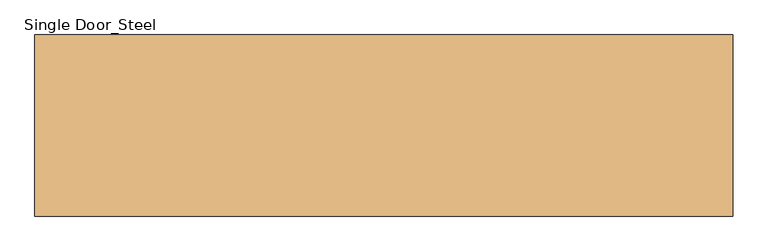
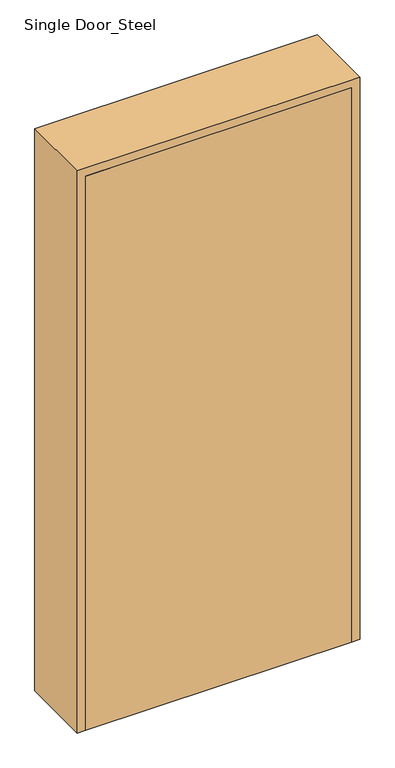
"""IFC4 building model written with IfcOpenShell, lengths in millimetres: door geometry, Single Door_Steel : H_DR_AR_B12_Single Door_Steel_W1000xH2100."""

from ifc_helpers import new_model, si_unit, origin, origin_with_axes, place, context, project, spatial, polyline, outline, extrude, faceted_brep, source, transform, mapped, element, save


def single_door_steel_02f153ad(model_context):
    return source(origin(), model_context, "Body", "SolidModel", [
        extrude(outline(polyline([(470.0, -130.0), (-470.0, -130.0), (-470.0, -95.0), (470.0, -95.0), (470.0, -130.0)])), origin_with_axes(), (0.0, 0.0, 1.0), 2070.0),
        faceted_brep([(470.0, -130.0, 0.0), (470.0, -95.0, 0.0), (450.0, -95.0, 0.0), (450.0, 95.0, 0.0), (470.0, 95.0, 0.0), (470.0, 130.0, 0.0), (500.0, 130.0, 0.0), (500.0, -130.0, 0.0), (500.0, -130.0, 2100.0), (-500.0, -130.0, 2100.0), (-500.0, -130.0, 0.0), (-470.0, -130.0, 0.0), (-470.0, -130.0, 2070.0), (470.0, -130.0, 2070.0), (500.0, 130.0, 2100.0), (470.0, 130.0, 2070.0), (-470.0, 130.0, 2070.0), (-470.0, 130.0, 0.0), (-500.0, 130.0, 0.0), (-500.0, 130.0, 2100.0), (470.0, 95.0, 2070.0), (450.0, 95.0, 2050.0), (-450.0, 95.0, 2050.0), (-450.0, 95.0, 0.0), (-470.0, 95.0, 0.0), (-470.0, 95.0, 2070.0), (450.0, -95.0, 2050.0), (470.0, -95.0, 2070.0), (-470.0, -95.0, 2070.0), (-470.0, -95.0, 0.0), (-450.0, -95.0, 0.0), (-450.0, -95.0, 2050.0)], [[[0, 1, 2, 3, 4, 5, 6, 7]], [[7, 8, 9, 10, 11, 12, 13, 0]], [[6, 14, 8, 7]], [[5, 15, 16, 17, 18, 19, 14, 6]], [[4, 20, 15, 5]], [[3, 21, 22, 23, 24, 25, 20, 4]], [[2, 26, 21, 3]], [[1, 27, 28, 29, 30, 31, 26, 2]], [[0, 13, 27, 1]], [[12, 11, 29, 28]], [[11, 10, 18, 17, 24, 23, 30, 29]], [[19, 18, 10, 9]], [[25, 24, 17, 16]], [[31, 30, 23, 22]], [[14, 19, 9, 8]], [[20, 25, 16, 15]], [[26, 31, 22, 21]], [[13, 12, 28, 27]]]),
    ])


if __name__ == "__main__":
    model = new_model("IFC4")
    model_context = context("Model", 3, world=origin())
    ifc_project = project(units=[si_unit("LENGTHUNIT", "METRE", prefix="MILLI")], contexts=[model_context])
    site = spatial("IfcSite", under=ifc_project)
    building = spatial("IfcBuilding", under=site)
    placement = place(None, origin())
    single_door_steel_shape = single_door_steel_02f153ad(model_context)
    element("IfcDoor", 1, ObjectType="Single Door_Steel : H_DR_AR_B12_Single Door_Steel_W1000xH2100", at=placement, inside=building, context=model_context, shape_type="MappedRepresentation", body=[
        mapped(single_door_steel_shape, transform((0.0, 0.0, 0.0), x_axis=(1.0, 0.0, 0.0), y_axis=(0.0, 1.0, 0.0), z_axis=(0.0, 0.0, 1.0))),
    ])
    save(model, "model.ifc")

# Revit data of these elements
# Type "Single Door_Steel : H_DR_AR_B12_Single Door_Steel_W1000xH2100"
#   Type Mark = "SD"
#   Analytic Construction = "<None>"
#   프레임 투영 외부. = 25 mm
#   프레임 투영 내부. = 25 mm
#   프레임 폭 = 75 mm
#   Height = 2100 mm
#   Width = 1000 mm
#   Define Thermal Properties by = 1
#   문 패널 = none
#   문 프레임 = none
#   Function = (empty or 0)
#   Wall Closure = (empty or 0)
